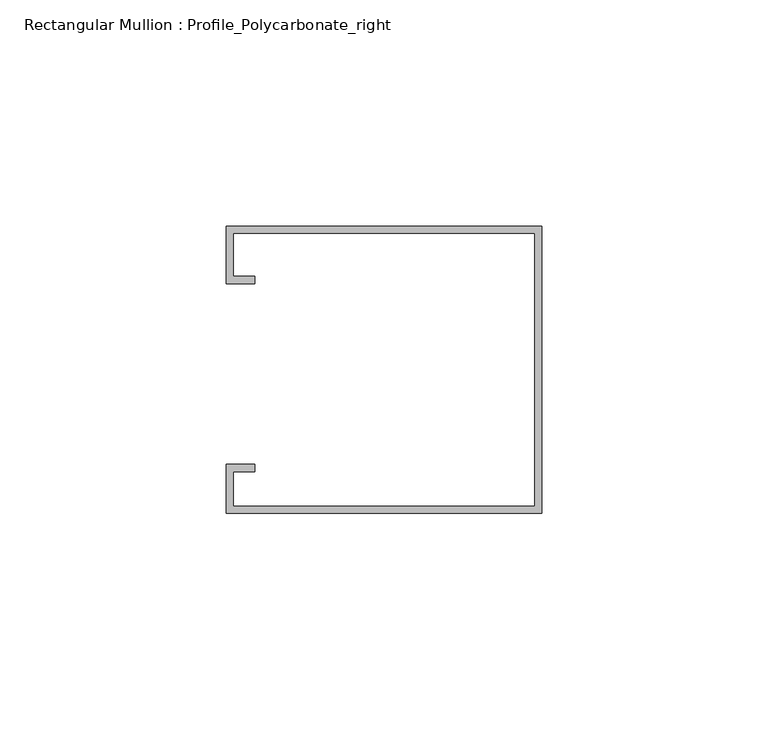
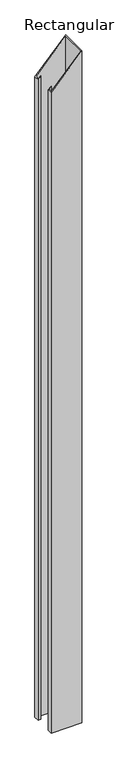
"""IFC4 building model written with IfcOpenShell, lengths in millimetres: member geometry, Rectangular Mullion : Profile_Polycarbonate_right."""

import ifcopenshell
import ifcopenshell.guid

model = None  # the IFC model being written
_history = None  # IfcOwnerHistory: only IFC2X3 demands one
_inside = {}  # id of a spatial element -> (the spatial element, [elements in it])
_under = {}  # id of a project, library or spatial element -> (it, [spatial elements below it])
_declared = {}  # id of a project -> (the project, [libraries it declares])
_typed = {}  # id of a type object -> (the type object, [elements of that type])
_made_of = {}  # id of a material, layer set ... -> (it, [elements and type objects made of it])


def new_model(schema):
    """Start an empty IFC model of exactly this schema.

    Asked for "IFC4X3", IfcOpenShell would pick the latest addendum, in which some entities
    have other attributes; the version numbers below select the first issue.
    IFC2X3 requires an IfcOwnerHistory on every rooted entity: one is made here for all.
    """
    global model, _history
    if schema == "IFC4X3":
        model = ifcopenshell.file(schema_version=(4, 3, 0, 0))
    else:
        model = ifcopenshell.file(schema=schema)
    _inside.clear()
    _under.clear()
    _declared.clear()
    _typed.clear()
    _made_of.clear()
    _history = None
    if model.schema == "IFC2X3":
        org = make("IfcOrganization", Name="unknown")
        user = make(
            "IfcPersonAndOrganization",
            ThePerson=make("IfcPerson", FamilyName="unknown"),
            TheOrganization=org,
        )
        app = make(
            "IfcApplication",
            ApplicationDeveloper=org,
            Version="unknown",
            ApplicationFullName="unknown",
            ApplicationIdentifier="unknown",
        )
        _history = make(
            "IfcOwnerHistory",
            OwningUser=user,
            OwningApplication=app,
            ChangeAction="ADDED",
            CreationDate=0,
        )
    return model


def make(cls, **values):
    """One entity of the class cls with the attributes given. An attribute that is None is left unset."""
    return model.create_entity(
        cls, **{name: value for name, value in values.items() if value is not None}
    )


def rooted(cls, **values):
    """An entity with a GlobalId (a new one), such as an element, a storey or a relation."""
    return make(cls, GlobalId=ifcopenshell.guid.new(), OwnerHistory=_history, **values)


def si_unit(unit_type, name, prefix=None):
    """IfcSIUnit, for example si_unit("LENGTHUNIT", "METRE", prefix="MILLI")."""
    return make("IfcSIUnit", UnitType=unit_type, Prefix=prefix, Name=name)


def assignment(units):
    """IfcUnitAssignment: the units of a project."""
    return None if units is None else make("IfcUnitAssignment", Units=units)


def point(xyz):
    """IfcCartesianPoint."""
    return None if xyz is None else make("IfcCartesianPoint", Coordinates=xyz)


def direction(xyz):
    """IfcDirection."""
    return None if xyz is None else make("IfcDirection", DirectionRatios=xyz)


def frame(location, z_axis=None, x_axis=None):
    """IfcAxis2Placement3D, a coordinate frame: its origin and axes. An axis left out is left unset."""
    return make(
        "IfcAxis2Placement3D",
        Location=point(location),
        Axis=direction(z_axis),
        RefDirection=direction(x_axis),
    )


def origin():
    """The frame at (0, 0, 0) with its axes left unset."""
    return frame((0.0, 0.0, 0.0))


def place(relative_to, where):
    """IfcLocalPlacement: puts the frame where relative to a parent placement (None: the world)."""
    return make(
        "IfcLocalPlacement", PlacementRelTo=relative_to, RelativePlacement=where
    )


def context(
    kind, dimensions, precision=None, world=None, true_north=None, identifier=None
):
    """IfcGeometricRepresentationContext, for example the 3D "Model" context."""
    return make(
        "IfcGeometricRepresentationContext",
        ContextIdentifier=identifier,
        ContextType=kind,
        CoordinateSpaceDimension=dimensions,
        Precision=precision,
        WorldCoordinateSystem=world,
        TrueNorth=true_north,
    )


def project(units=None, contexts=None):
    """IfcProject with its units and contexts."""
    return rooted(
        "IfcProject",
        Name="project",
        RepresentationContexts=contexts,
        UnitsInContext=assignment(units),
    )


def spatial(cls, under=None, at=None, **own):
    """A site, building, storey or space (cls), placed at a placement, below another one or the project."""
    s = rooted(cls, ObjectPlacement=at, **own)
    if under is not None:
        _under.setdefault(under.id(), (under, []))[1].append(s)
    return s


def faces_of(points, faces, orient=None, outer=None):
    """IfcFace entities. A face is a list of loops; a loop is a list of indices into points, from 0.

    orient and outer hold one flag for each loop. By default every Orientation is true, the
    first loop of a face is its IfcFaceOuterBound and the others are IfcFaceBound.
    """
    made = []
    for i, loops in enumerate(faces):
        bounds = []
        for j, loop in enumerate(loops):
            is_outer = j == 0 if outer is None else outer[i][j]
            bounds.append(
                make(
                    "IfcFaceOuterBound" if is_outer else "IfcFaceBound",
                    Bound=make("IfcPolyLoop", Polygon=[points[k] for k in loop]),
                    Orientation=True if orient is None else orient[i][j],
                )
            )
        made.append(make("IfcFace", Bounds=bounds))
    return made


def faceted_brep(points, faces, orient=None, outer=None, voids=None):
    """IfcFacetedBrep: a solid bounded by flat faces; with voids (closed shells), ...WithVoids."""
    shared = [point(p) for p in points]
    hull = make("IfcClosedShell", CfsFaces=faces_of(shared, faces, orient, outer))
    if voids is None:
        return make("IfcFacetedBrep", Outer=hull)
    return make(
        "IfcFacetedBrepWithVoids",
        Outer=hull,
        Voids=[
            make(cls, CfsFaces=faces_of(shared, fs, o, b)) for cls, fs, o, b in voids
        ],
    )


def shape(context_of_items, identifier, shape_type, items):
    """IfcShapeRepresentation: the items that make up one representation, for example the "Body"."""
    return make(
        "IfcShapeRepresentation",
        ContextOfItems=context_of_items,
        RepresentationIdentifier=identifier,
        RepresentationType=shape_type,
        Items=items,
    )


def source(mapping_origin, context_of_items, identifier, shape_type, items):
    """IfcRepresentationMap: a shape defined once, which mapped items show again and again."""
    return make(
        "IfcRepresentationMap",
        MappingOrigin=mapping_origin,
        MappedRepresentation=shape(context_of_items, identifier, shape_type, items),
    )


def transform(
    local_origin,
    x_axis=None,
    y_axis=None,
    z_axis=None,
    scale=None,
    scale2=None,
    scale3=None,
    uniform=True,
):
    """IfcCartesianTransformationOperator3D, or its non-uniform kind. x_axis, y_axis, z_axis: its Axis1, 2, 3."""
    if uniform:
        return make(
            "IfcCartesianTransformationOperator3D",
            Axis1=direction(x_axis),
            Axis2=direction(y_axis),
            LocalOrigin=point(local_origin),
            Scale=scale,
            Axis3=direction(z_axis),
        )
    return make(
        "IfcCartesianTransformationOperator3DnonUniform",
        Axis1=direction(x_axis),
        Axis2=direction(y_axis),
        LocalOrigin=point(local_origin),
        Scale=scale,
        Axis3=direction(z_axis),
        Scale2=scale2,
        Scale3=scale3,
    )


def mapped(mapping_source, mapping_target):
    """IfcMappedItem: shows the shape of a source again, moved by a transform."""
    return make(
        "IfcMappedItem", MappingSource=mapping_source, MappingTarget=mapping_target
    )


def made_of(thing, what):
    """Note that an element or type object is made of a material, layer set ...; save() writes the relation."""
    if what is not None:
        _made_of.setdefault(what.id(), (what, []))[1].append(thing)
    return thing


def element(
    cls,
    number,
    at=None,
    inside=None,
    cuts=None,
    type_object=None,
    material=None,
    context=None,
    identifier="Body",
    shape_type=None,
    held_by="IfcProductDefinitionShape",
    body=None,
    shapes=None,
    **own,
):
    """One element of the class cls, such as IfcWall. Its Tag is "e" and its number.

    at: its placement. inside: the storey or other place that contains it. cuts: it is an
    opening in that element (IfcRelVoidsElement). A single representation is given by context,
    identifier, shape_type and body (its items); several are given by shapes. held_by: the class
    of the entity that holds the representations. save() writes the other relations.
    """
    e = rooted(cls, Tag="e%d" % number, ObjectPlacement=at, **own)
    if body is not None:
        shapes = [shape(context, identifier, shape_type, body)]
    if shapes is not None:
        e.Representation = make(held_by, Representations=shapes)
    if inside is not None:
        _inside.setdefault(inside.id(), (inside, []))[1].append(e)
    if cuts is not None:
        rooted(
            "IfcRelVoidsElement", RelatingBuildingElement=cuts, RelatedOpeningElement=e
        )
    if type_object is not None:
        _typed.setdefault(type_object.id(), (type_object, []))[1].append(e)
    return made_of(e, material)


def aggregate(whole, parts):
    """IfcRelAggregates: a whole, such as a stair, and the parts it consists of."""
    return rooted("IfcRelAggregates", RelatingObject=whole, RelatedObjects=parts)


def save(model, path):
    """Write the relations noted so far, then the file.

    IfcRelAggregates (storeys below a building ...), IfcRelContainedInSpatialStructure (elements
    in a storey), IfcRelDefinesByType, IfcRelAssociatesMaterial and IfcRelDeclares: one each for
    every whole, place, type object, material and project.
    """
    for whole, parts in _under.values():
        aggregate(whole, parts)
    for where, things in _inside.values():
        rooted(
            "IfcRelContainedInSpatialStructure",
            RelatedElements=things,
            RelatingStructure=where,
        )
    for kind, things in _typed.values():
        rooted("IfcRelDefinesByType", RelatedObjects=things, RelatingType=kind)
    for what, things in _made_of.values():
        rooted("IfcRelAssociatesMaterial", RelatedObjects=things, RelatingMaterial=what)
    for by, libraries in _declared.values():
        rooted("IfcRelDeclares", RelatingContext=by, RelatedDefinitions=libraries)
    model.write(path)


def rectangular_mullion_profile_polycarbonate_right_84cbc30a(model_context):
    return source(origin(), model_context, "Body", "Brep", [
        faceted_brep([(0.0, 32.7, -1614.090625), (0.0, -30.8, -1614.090625), (-69.85, -30.8, -1614.090625), (-69.85, -20.0, -1614.090625), (-63.5, -20.0, -1614.090625), (-63.5, -21.5875, -1614.090625), (-68.2625, -21.5875, -1614.090625), (-68.2625, -29.2125, -1614.090625), (-1.5875, -29.2125, -1614.090625), (-1.5875, 31.1125, -1614.090625), (-68.2625, 31.1125, -1614.090625), (-68.2625, 21.5875, -1614.090625), (-63.5, 21.5875, -1614.090625), (-63.5, 20.0, -1614.090625), (-69.85, 20.0, -1614.090625), (-69.85, 32.7, -1614.090625), (-69.85, 32.7, -75.9129484), (0.0, 32.7, 0.0), (-69.85, 20.0, -75.9129484), (-63.5, 20.0, -69.0117713), (-63.5, 21.5875, -69.0117713), (-68.2625, 21.5875, -74.1876542), (-68.2625, 31.1125, -74.1876542), (-1.5875, 31.1125, -1.7252943), (-1.5875, -29.2125, -1.7252943), (-68.2625, -29.2125, -74.1876542), (-68.2625, -21.5875, -74.1876542), (-63.5, -21.5875, -69.0117713), (-63.5, -20.0, -69.0117713), (-69.85, -20.0, -75.9129484), (-69.85, -30.8, -75.9129484), (0.0, -30.8, 0.0)], [[[0, 1, 2, 3, 4, 5, 6, 7, 8, 9, 10, 11, 12, 13, 14, 15]], [[16, 17, 0, 15]], [[18, 16, 15, 14]], [[19, 18, 14, 13]], [[20, 19, 13, 12]], [[21, 20, 12, 11]], [[22, 21, 11, 10]], [[23, 22, 10, 9]], [[24, 23, 9, 8]], [[25, 24, 8, 7]], [[26, 25, 7, 6]], [[27, 26, 6, 5]], [[28, 27, 5, 4]], [[29, 28, 4, 3]], [[30, 29, 3, 2]], [[31, 30, 2, 1]], [[17, 31, 1, 0]], [[17, 16, 18, 19, 20, 21, 22, 23, 24, 25, 26, 27, 28, 29, 30, 31]]]),
    ])


if __name__ == "__main__":
    model = new_model("IFC4")
    model_context = context("Model", 3, world=origin())
    ifc_project = project(units=[si_unit("LENGTHUNIT", "METRE", prefix="MILLI")], contexts=[model_context])
    site = spatial("IfcSite", under=ifc_project)
    building = spatial("IfcBuilding", under=site)
    placement = place(None, origin())
    rectangular_mullion_profile_polycarbonate_right_shape = rectangular_mullion_profile_polycarbonate_right_84cbc30a(model_context)
    element("IfcMember", 1, ObjectType="Rectangular Mullion : Profile_Polycarbonate_right", at=placement, inside=building, context=model_context, shape_type="MappedRepresentation", body=[
        mapped(rectangular_mullion_profile_polycarbonate_right_shape, transform((0.0, 0.0, 0.0), x_axis=(1.0, 0.0, 0.0), y_axis=(0.0, 1.0, 0.0), z_axis=(0.0, 0.0, 1.0))),
    ])
    save(model, "model.ifc")

# Revit data of these elements
# Type "Rectangular Mullion : Profile_Polycarbonate_right"
#   built-in parameter 1007322 = 0.208333 (stored number, unit not read)
#   built-in parameter 1007321 = 0 (stored number, unit not read)
#   built-in parameter 1007320 = 0.00520833 (stored number, unit not read)
# Element 1 (IfcMember, "Rectangular Mullion : Profile_Polycarbonate_right")
#   Materials on its faces: "ALUMINUM PROFILE AT POLYCARBONATE PANEL"
# Materials
#   "ALUMINUM PROFILE AT POLYCARBONATE PANEL": class "Metal", colour RGB 244 244 244, transparency 0, Description = "Aluminum 6061", Cost = 0
